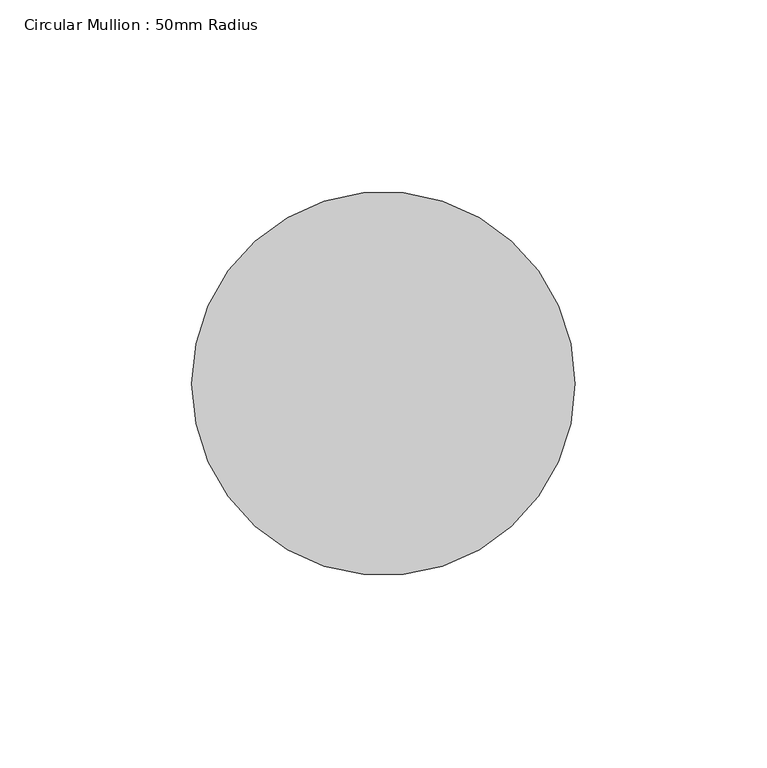
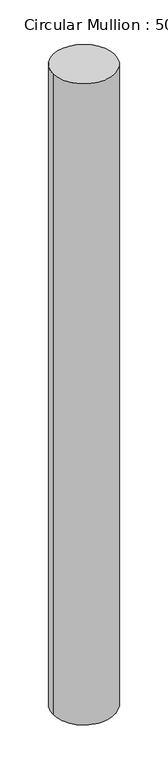
"""IFC4 building model written with IfcOpenShell, lengths in millimetres: member geometry, Circular Mullion : 50mm Radius."""

from ifc_helpers import new_model, si_unit, frame, origin, place, context, project, spatial, ellipse_curve, source, transform, mapped, element, save
from ifc_brep_helpers import plane_surface, cylinder_surface, advanced_brep


def circular_mullion_50mm_radius_2e630b8b(model_context):
    return source(origin(), model_context, "Body", "AdvancedBrep", [
        advanced_brep(
        [(-100.0, 0.0, 1.3689964), (0.0, 0.0, 0.0), (0.0, 0.0, -1096.3771252), (-100.0, 0.0, -1097.8158758)],
        [
            (0, 1, ellipse_curve(frame((-50.0, 0.0, 0.6844982), z_axis=(-0.013685580654970499, -0.02128295089280164, -0.999679819183838), x_axis=(-0.5406874235209076, -0.8408429407028127, 0.025303342003953143)), 50.0160142, 50.0)),
            (1, 2),
            (2, 3, ellipse_curve(frame((-50.0, 0.0, -1097.0965005), z_axis=(-0.014382418359250162, -0.022366628890422745, 0.9996463774526558), x_axis=(0.5406693362061957, 0.8408148124531165, 0.02659172889795371)), 50.0176874, 50.0)),
            (3, 0),
            (1, 0, ellipse_curve(frame((-50.0, 0.0, 0.6844982), z_axis=(-0.013685580654970499, -0.02128295089280164, -0.999679819183838), x_axis=(-0.5406874235209076, -0.8408429407028127, 0.025303342003953143)), 50.0160142, 50.0)),
            (3, 2, ellipse_curve(frame((-50.0, 0.0, -1097.0965005), z_axis=(-0.014382418359250162, -0.022366628890422745, 0.9996463774526558), x_axis=(0.5406693362061957, 0.8408148124531165, 0.02659172889795371)), 50.0176874, 50.0)),
        ],
        [
            cylinder_surface(frame((-50.0, 0.0, 0.0), z_axis=(0.0, 0.0, 1.0), x_axis=(1.0, 0.0, 0.0)), 50.0),
            plane_surface(frame((-256.3710134, 164.8543099, 0.0), z_axis=(0.013685580654970499, 0.02128295089280164, 0.999679819183838), x_axis=(0.540687423520907, 0.840842940702813, -0.02530334200395491))),
            plane_surface(frame((-256.3710134, 164.8543099, -1096.3771252), z_axis=(0.014382418359250162, 0.022366628890422745, -0.9996463774526558), x_axis=(0.5406693362061956, 0.8408148124531165, 0.026591728897956024))),
        ],
        [
            (0, [[1, 2, 3, 4]]),
            (0, [[5, -4, 6, -2]]),
            (1, [[-1, -5]]),
            (2, [[-6, -3]]),
        ],
    ),
    ])


if __name__ == "__main__":
    model = new_model("IFC4")
    model_context = context("Model", 3, world=origin())
    ifc_project = project(units=[si_unit("LENGTHUNIT", "METRE", prefix="MILLI")], contexts=[model_context])
    site = spatial("IfcSite", under=ifc_project)
    building = spatial("IfcBuilding", under=site)
    placement = place(None, origin())
    circular_mullion_50mm_radius_shape = circular_mullion_50mm_radius_2e630b8b(model_context)
    element("IfcMember", 1, ObjectType="Circular Mullion : 50mm Radius", at=placement, inside=building, context=model_context, shape_type="MappedRepresentation", body=[
        mapped(circular_mullion_50mm_radius_shape, transform((0.0, 0.0, 0.0), x_axis=(1.0, 0.0, 0.0), y_axis=(0.0, 1.0, 0.0), z_axis=(0.0, 0.0, 1.0))),
    ])
    save(model, "model.ifc")

# Revit data of these elements
# Type "Circular Mullion : 50mm Radius"
#   built-in parameter 1007350 = 0.164042 (stored number, unit not read)
# Element 1 (IfcMember, "Circular Mullion : 50mm Radius")
#   Materials on its faces: "Aluminium"
# Materials
#   "Aluminium": class "Metal", colour RGB 247 247 247, transparency 0, Description = "Aluminium 6061", Cost = 0
